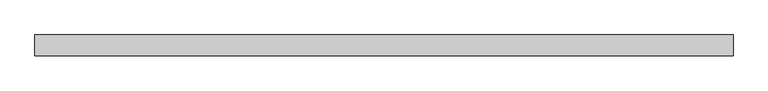
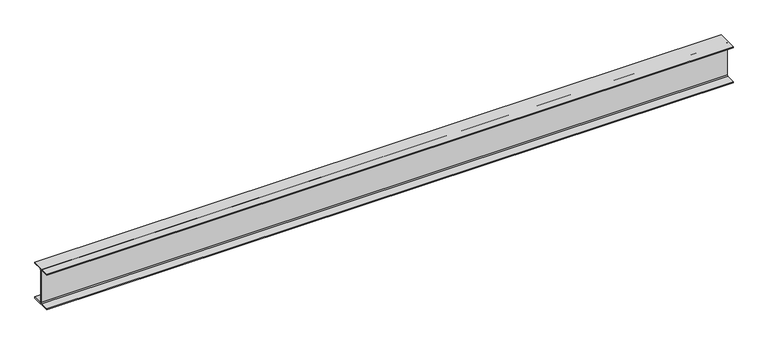
"""IFC4 building model written with IfcOpenShell, lengths in millimetres: beam geometry, Old_Steel Beam_H-KSD3502 : H_SB_ASB_H-482×300x11x15."""

from ifc_helpers import new_model, si_unit, point, frame, frame_2d, origin, place, context, project, spatial, polyline, circle_curve, trimmed, segment, composite_curve, outline, extrude, source, transform, mapped, element, save


def beam_de3997fd(model_context):
    return source(origin(), model_context, "Body", "SweptSolid", [
        extrude(outline(composite_curve([segment(polyline([(82.5, -141.5), (82.5, -151.7), (-82.5, -151.7), (-82.5, -141.5), (-11.9, -141.5)]), True, "CONTINUOUS"), segment(trimmed(circle_curve(frame_2d((-11.9, -132.6)), 8.9), [point((-11.9, -141.5))], [point((-3.0, -132.6))], True, "CARTESIAN"), True, "CONTINUOUS"), segment(polyline([(-3.0, -132.6), (-3.0, 132.6)]), True, "CONTINUOUS"), segment(trimmed(circle_curve(frame_2d((-11.9, 132.6)), 8.9), [point((-3.0, 132.6))], [point((-11.9, 141.5))], True, "CARTESIAN"), True, "CONTINUOUS"), segment(polyline([(-11.9, 141.5), (-82.5, 141.5), (-82.5, 151.7), (82.5, 151.7), (82.5, 141.5), (11.9, 141.5)]), True, "CONTINUOUS"), segment(trimmed(circle_curve(frame_2d((11.9, 132.6)), 8.9), [point((11.9, 141.5))], [point((3.0, 132.6))], True, "CARTESIAN"), True, "CONTINUOUS"), segment(polyline([(3.0, 132.6), (3.0, -132.6)]), True, "CONTINUOUS"), segment(trimmed(circle_curve(frame_2d((11.9, -132.6)), 8.9), [point((3.0, -132.6))], [point((11.9, -141.5))], True, "CARTESIAN"), True, "CONTINUOUS"), segment(polyline([(11.9, -141.5), (82.5, -141.5)]), True, "CONTINUOUS")], self_intersect=False)), frame((-2837.3, 0.0, 0.0), z_axis=(1.0, 0.0, 0.0), x_axis=(0.0, 1.0, 0.0)), (0.0, 0.0, 1.0), 5474.6),
    ])


if __name__ == "__main__":
    model = new_model("IFC4")
    model_context = context("Model", 3, world=origin())
    ifc_project = project(units=[si_unit("LENGTHUNIT", "METRE", prefix="MILLI")], contexts=[model_context])
    site = spatial("IfcSite", under=ifc_project)
    building = spatial("IfcBuilding", under=site)
    placement = place(None, origin())
    beam_shape = beam_de3997fd(model_context)
    element("IfcBeam", 1, ObjectType="Old_Steel Beam_H-KSD3502 : H_SB_ASB_H-482×300x11x15", at=placement, inside=building, context=model_context, shape_type="MappedRepresentation", body=[
        mapped(beam_shape, transform((0.0, 0.0, 0.0), x_axis=(1.0, 0.0, 0.0), y_axis=(0.0, 1.0, 0.0), z_axis=(0.0, 0.0, 1.0))),
    ])
    save(model, "model.ifc")

# Revit data of these elements
# Type "Old_Steel Beam_H-KSD3502 : H_SB_ASB_H-482×300x11x15"
#   Width = 30.0 cm
#   Web Thickness = 1.1 cm
#   Web Fillet = 2.6 cm
#   Warping Constant = 3680250.0 cm⁶
#   Torsional Moment of Inertia = 88.2192 cm⁴
#   Torsional Modulus = 1.0 cm³
#   Section Area = 145.5 cm²
#   Plastic Modulus weak axis = 695.0 cm³
#   Plastic Modulus strong axis = 2790.0 cm³
#   Perimeter = 2.10 m²/m
#   Nominal Weight = 114.00 kgf/m
#   Moment of Inertia weak axis = 6760.00 cm⁴
#   Moment of Inertia strong axis = 60400.00 cm⁴
#   Height = 48.2 cm
#   Flange Thickness = 1.5 cm
#   Elastic Modulus weak axis = 451.0 cm³
#   Elastic Modulus strong axis = 2500.0 cm³
#   Centroid Vertical = 24.1 cm
#   Centroid Horizontal = 15.0 cm
#   Length [instance default] = 1.5240 m
#   Structural Material [instance default] = Steel, 45-345
#   Assembly Code = ""
# Element 1 (IfcBeam, "Old_Steel Beam_H-KSD3502 : H_SB_ASB_H-482×300x11x15")
#   Structural Material = none
# Materials
#   "Steel, 45-345": class "Metal", colour RGB 189 187 185, transparency 0, Description = "Steel 345 MPa", Cost = 0
